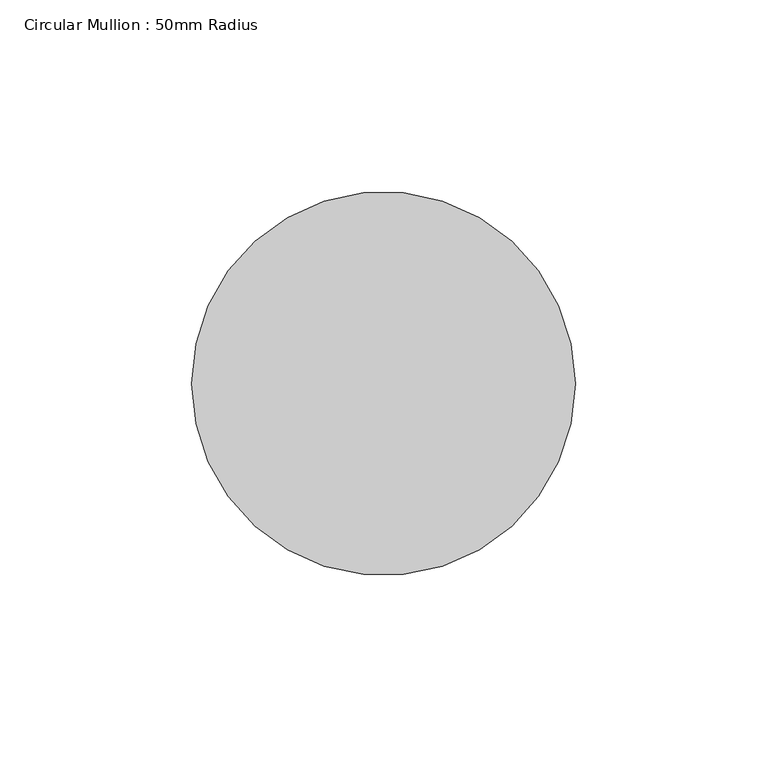
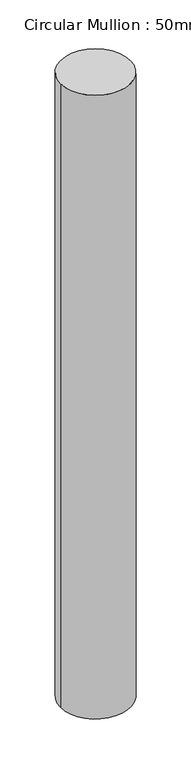
"""IFC4 building model written with IfcOpenShell, lengths in millimetres: member geometry, Circular Mullion : 50mm Radius."""

from ifc_helpers import new_model, si_unit, point, frame, origin, origin_2d, place, context, project, spatial, circle_curve, trimmed, segment, composite_curve, outline, extrude, source, transform, mapped, element, save


def circular_mullion_50mm_radius_b5ace9f3(model_context):
    return source(origin(), model_context, "Body", "SweptSolid", [
        extrude(outline(composite_curve([segment(trimmed(circle_curve(origin_2d(), 50.0), [point((50.0, 0.0))], [point((-50.0, 0.0))], False, "CARTESIAN"), True, "CONTINUOUS"), segment(trimmed(circle_curve(origin_2d(), 50.0), [point((-50.0, 0.0))], [point((50.0, 0.0))], False, "CARTESIAN"), True, "CONTINUOUS")], self_intersect=False)), frame((0.0, 0.0, -941.4197249), z_axis=(0.0, 0.0, 1.0), x_axis=(1.0, 0.0, 0.0)), (0.0, 0.0, 1.0), 941.4197249),
    ])


if __name__ == "__main__":
    model = new_model("IFC4")
    model_context = context("Model", 3, world=origin())
    ifc_project = project(units=[si_unit("LENGTHUNIT", "METRE", prefix="MILLI")], contexts=[model_context])
    site = spatial("IfcSite", under=ifc_project)
    building = spatial("IfcBuilding", under=site)
    placement = place(None, origin())
    circular_mullion_50mm_radius_shape = circular_mullion_50mm_radius_b5ace9f3(model_context)
    element("IfcMember", 1, ObjectType="Circular Mullion : 50mm Radius", at=placement, inside=building, context=model_context, shape_type="MappedRepresentation", body=[
        mapped(circular_mullion_50mm_radius_shape, transform((0.0, 0.0, 0.0), x_axis=(1.0, 0.0, 0.0), y_axis=(0.0, 1.0, 0.0), z_axis=(0.0, 0.0, 1.0))),
    ])
    save(model, "model.ifc")

# Revit data of these elements
# Type "Circular Mullion : 50mm Radius"
#   built-in parameter 1007350 = 0.164042 (stored number, unit not read)
# Element 1 (IfcMember, "Circular Mullion : 50mm Radius")
#   Materials on its faces: "Aluminium"
# Materials
#   "Aluminium": class "Metal", colour RGB 247 247 247, transparency 0, Description = "Aluminium 6061", Cost = 0
